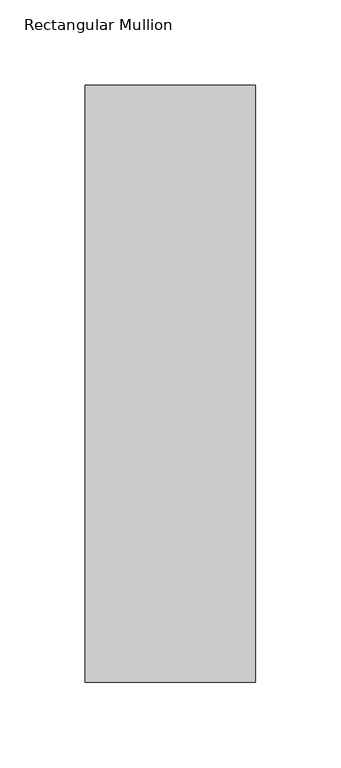
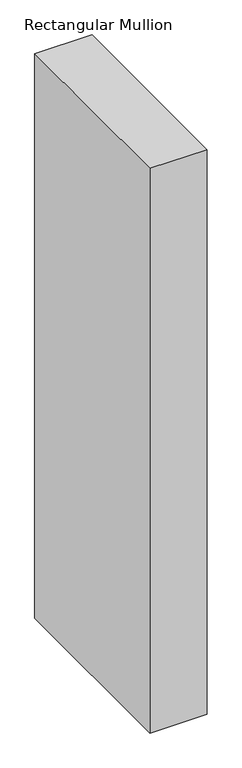
"""IFC4 building model written with IfcOpenShell, lengths in millimetres: member geometry, Rectangular Mullion : WWm-100x350-100mmOffset."""

from ifc_helpers import new_model, si_unit, frame, origin, place, context, project, spatial, polyline, outline, extrude, source, transform, mapped, element, save


def rectangular_mullion_50874f85(model_context):
    return source(origin(), model_context, "Body", "SweptSolid", [
        extrude(outline(polyline([(0.0, 175.0), (0.0, -175.0), (-100.0, -175.0), (-100.0, 175.0), (0.0, 175.0)])), frame((0.0, 0.0, -1045.4500931), z_axis=(0.0, 0.0, 1.0), x_axis=(1.0, 0.0, 0.0)), (0.0, 0.0, 1.0), 1045.4500931),
    ])


if __name__ == "__main__":
    model = new_model("IFC4")
    model_context = context("Model", 3, world=origin())
    ifc_project = project(units=[si_unit("LENGTHUNIT", "METRE", prefix="MILLI")], contexts=[model_context])
    site = spatial("IfcSite", under=ifc_project)
    building = spatial("IfcBuilding", under=site)
    placement = place(None, origin())
    rectangular_mullion_shape = rectangular_mullion_50874f85(model_context)
    element("IfcMember", 1, ObjectType="Rectangular Mullion : WWm-100x350-100mmOffset", at=placement, inside=building, context=model_context, shape_type="MappedRepresentation", body=[
        mapped(rectangular_mullion_shape, transform((0.0, 0.0, 0.0), x_axis=(1.0, 0.0, 0.0), y_axis=(0.0, 1.0, 0.0), z_axis=(0.0, 0.0, 1.0))),
    ])
    save(model, "model.ifc")

# Revit data of these elements
# Type "Rectangular Mullion : WWm-100x350-100mmOffset"
#   built-in parameter 1007304 = 1.14829 (stored number, unit not read)
#   built-in parameter 1007301 = 0.164042 (stored number, unit not read)
#   built-in parameter 1007300 = 0.164042 (stored number, unit not read)
# Element 1 (IfcMember, "Rectangular Mullion : WWm-100x350-100mmOffset")
#   Materials on its faces: "WW-EC-RGB-Mullion"
# Materials
#   "WW-EC-RGB-Mullion": class "Generic", colour RGB 255 255 255, transparency 0, Comments = "If region requests black mullions, switch asset color to RGB 25-25-25", Description = "Generic Color", Cost = 0
